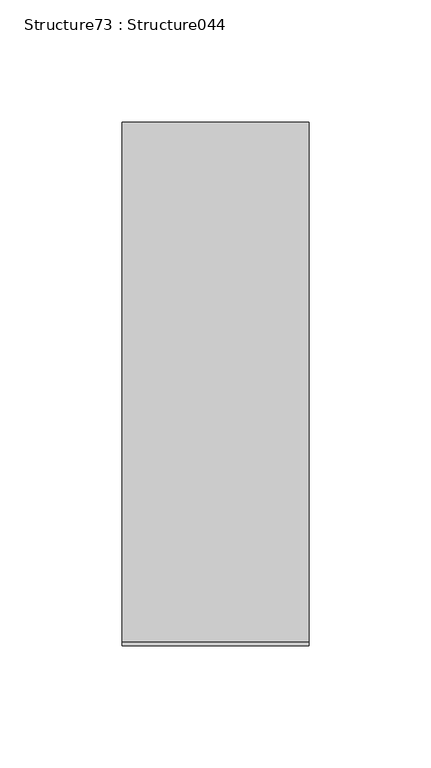
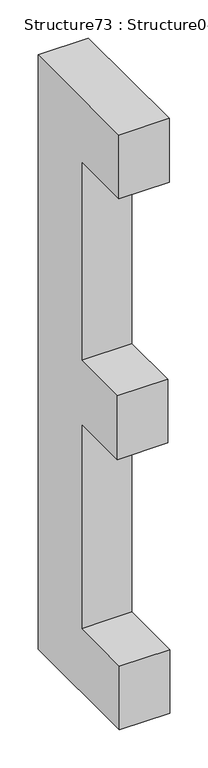
"""IFC4 building model written with IfcOpenShell, lengths in millimetres: proxy geometry, Structure73 : Structure044."""

from ifc_helpers import new_model, si_unit, frame, origin, place, context, project, spatial, polyline, outline, extrude, source, transform, mapped, element, save


def structure73_structure044_2a1b00d1(model_context):
    return source(origin(), model_context, "Body", "SweptSolid", [
        extrude(outline(polyline([(281940.4785876, 4480.4419946), (281940.4785876, 3528.5825142), (281726.990168, 3528.5825142), (281726.990168, 3630.5630275), (281826.2424512, 3630.5630275), (281826.2424512, 3958.2800261), (281732.4308837, 3958.2800261), (281732.4308837, 4060.2611693), (281826.2424512, 4060.2611693), (281826.2424512, 4378.4602217), (281728.3460959, 4378.4602217), (281728.3460959, 4480.4419946), (281940.4785876, 4480.4419946)])), frame((-59031.6926606, 0.0, 0.0), z_axis=(1.0, 0.0, 0.0), x_axis=(0.0, 1.0, 0.0)), (0.0, 0.0, 1.0), 76.2),
    ])


if __name__ == "__main__":
    model = new_model("IFC4")
    model_context = context("Model", 3, world=origin())
    ifc_project = project(units=[si_unit("LENGTHUNIT", "METRE", prefix="MILLI")], contexts=[model_context])
    site = spatial("IfcSite", under=ifc_project)
    building = spatial("IfcBuilding", under=site)
    placement = place(None, origin())
    structure73_structure044_shape = structure73_structure044_2a1b00d1(model_context)
    element("IfcBuildingElementProxy", 1, Name="Structure73 : Structure044", ObjectType="Structure73 : Structure044", at=placement, inside=building, context=model_context, shape_type="MappedRepresentation", body=[
        mapped(structure73_structure044_shape, transform((0.0, 0.0, 0.0), x_axis=(1.0, 0.0, 0.0), y_axis=(0.0, 1.0, 0.0), z_axis=(0.0, 0.0, 1.0))),
    ])
    save(model, "model.ifc")

# Revit data of these elements
# Type "Structure73 : Structure044"
#   NameOverride = "Structure044"
# Element 1 (IfcBuildingElementProxy, "Structure73 : Structure044")
#   Materials on its faces: "BRUSHED ALUM. LETTERING"
# Materials
#   "BRUSHED ALUM. LETTERING": class "Unassigned", colour RGB 169 181 186, transparency 0, Cost = 0
